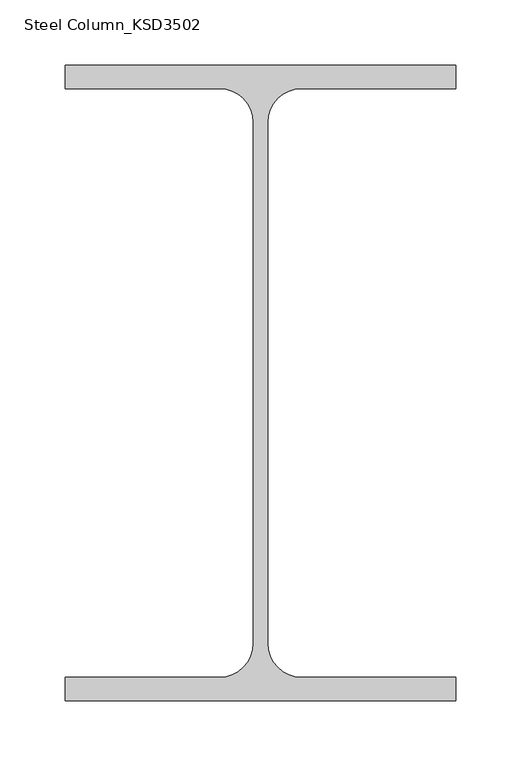
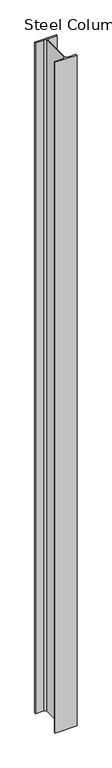
"""IFC4 building model written with IfcOpenShell, lengths in millimetres: column geometry, Steel Column_KSD3502 : H_SC_ASC_H-488×300x11x18."""

import ifcopenshell
import ifcopenshell.guid

model = None  # the IFC model being written
_history = None  # IfcOwnerHistory: only IFC2X3 demands one
_inside = {}  # id of a spatial element -> (the spatial element, [elements in it])
_under = {}  # id of a project, library or spatial element -> (it, [spatial elements below it])
_declared = {}  # id of a project -> (the project, [libraries it declares])
_typed = {}  # id of a type object -> (the type object, [elements of that type])
_made_of = {}  # id of a material, layer set ... -> (it, [elements and type objects made of it])


def new_model(schema):
    """Start an empty IFC model of exactly this schema.

    Asked for "IFC4X3", IfcOpenShell would pick the latest addendum, in which some entities
    have other attributes; the version numbers below select the first issue.
    IFC2X3 requires an IfcOwnerHistory on every rooted entity: one is made here for all.
    """
    global model, _history
    if schema == "IFC4X3":
        model = ifcopenshell.file(schema_version=(4, 3, 0, 0))
    else:
        model = ifcopenshell.file(schema=schema)
    _inside.clear()
    _under.clear()
    _declared.clear()
    _typed.clear()
    _made_of.clear()
    _history = None
    if model.schema == "IFC2X3":
        org = make("IfcOrganization", Name="unknown")
        user = make(
            "IfcPersonAndOrganization",
            ThePerson=make("IfcPerson", FamilyName="unknown"),
            TheOrganization=org,
        )
        app = make(
            "IfcApplication",
            ApplicationDeveloper=org,
            Version="unknown",
            ApplicationFullName="unknown",
            ApplicationIdentifier="unknown",
        )
        _history = make(
            "IfcOwnerHistory",
            OwningUser=user,
            OwningApplication=app,
            ChangeAction="ADDED",
            CreationDate=0,
        )
    return model


def make(cls, **values):
    """One entity of the class cls with the attributes given. An attribute that is None is left unset."""
    return model.create_entity(
        cls, **{name: value for name, value in values.items() if value is not None}
    )


def rooted(cls, **values):
    """An entity with a GlobalId (a new one), such as an element, a storey or a relation."""
    return make(cls, GlobalId=ifcopenshell.guid.new(), OwnerHistory=_history, **values)


def si_unit(unit_type, name, prefix=None):
    """IfcSIUnit, for example si_unit("LENGTHUNIT", "METRE", prefix="MILLI")."""
    return make("IfcSIUnit", UnitType=unit_type, Prefix=prefix, Name=name)


def assignment(units):
    """IfcUnitAssignment: the units of a project."""
    return None if units is None else make("IfcUnitAssignment", Units=units)


def point(xyz):
    """IfcCartesianPoint."""
    return None if xyz is None else make("IfcCartesianPoint", Coordinates=xyz)


def direction(xyz):
    """IfcDirection."""
    return None if xyz is None else make("IfcDirection", DirectionRatios=xyz)


def frame(location, z_axis=None, x_axis=None):
    """IfcAxis2Placement3D, a coordinate frame: its origin and axes. An axis left out is left unset."""
    return make(
        "IfcAxis2Placement3D",
        Location=point(location),
        Axis=direction(z_axis),
        RefDirection=direction(x_axis),
    )


def frame_2d(location, x_axis=None):
    """IfcAxis2Placement2D, a coordinate frame in the plane: its origin and x axis."""
    return make(
        "IfcAxis2Placement2D", Location=point(location), RefDirection=direction(x_axis)
    )


def origin():
    """The frame at (0, 0, 0) with its axes left unset."""
    return frame((0.0, 0.0, 0.0))


def place(relative_to, where):
    """IfcLocalPlacement: puts the frame where relative to a parent placement (None: the world)."""
    return make(
        "IfcLocalPlacement", PlacementRelTo=relative_to, RelativePlacement=where
    )


def context(
    kind, dimensions, precision=None, world=None, true_north=None, identifier=None
):
    """IfcGeometricRepresentationContext, for example the 3D "Model" context."""
    return make(
        "IfcGeometricRepresentationContext",
        ContextIdentifier=identifier,
        ContextType=kind,
        CoordinateSpaceDimension=dimensions,
        Precision=precision,
        WorldCoordinateSystem=world,
        TrueNorth=true_north,
    )


def project(units=None, contexts=None):
    """IfcProject with its units and contexts."""
    return rooted(
        "IfcProject",
        Name="project",
        RepresentationContexts=contexts,
        UnitsInContext=assignment(units),
    )


def spatial(cls, under=None, at=None, **own):
    """A site, building, storey or space (cls), placed at a placement, below another one or the project."""
    s = rooted(cls, ObjectPlacement=at, **own)
    if under is not None:
        _under.setdefault(under.id(), (under, []))[1].append(s)
    return s


def polyline(points):
    """IfcPolyline through the points."""
    return make("IfcPolyline", Points=[point(p) for p in points])


def circle_curve(where, radius):
    """IfcCircle in the frame where."""
    return make("IfcCircle", Position=where, Radius=radius)


def trimmed(basis, trim1, trim2, sense, master):
    """IfcTrimmedCurve: the piece of a basis curve between two trims."""
    return make(
        "IfcTrimmedCurve",
        BasisCurve=basis,
        Trim1=trim1,
        Trim2=trim2,
        SenseAgreement=sense,
        MasterRepresentation=master,
    )


def segment(curve, same_sense, transition):
    """IfcCompositeCurveSegment."""
    return make(
        "IfcCompositeCurveSegment",
        Transition=transition,
        SameSense=same_sense,
        ParentCurve=curve,
    )


def composite_curve(segments, self_intersect=None):
    """IfcCompositeCurve: segments joined end to end."""
    return make("IfcCompositeCurve", Segments=segments, SelfIntersect=self_intersect)


def outline(outer, holes=None, kind="AREA"):
    """IfcArbitraryClosedProfileDef: a profile drawn as a closed curve; with holes, ...WithVoids."""
    if holes is None:
        return make("IfcArbitraryClosedProfileDef", ProfileType=kind, OuterCurve=outer)
    return make(
        "IfcArbitraryProfileDefWithVoids",
        ProfileType=kind,
        OuterCurve=outer,
        InnerCurves=holes,
    )


def extrude(swept, where, along, depth):
    """IfcExtrudedAreaSolid: the profile swept, set in the frame where, extruded along a direction by depth."""
    return make(
        "IfcExtrudedAreaSolid",
        SweptArea=swept,
        Position=where,
        ExtrudedDirection=direction(along),
        Depth=depth,
    )


def shape(context_of_items, identifier, shape_type, items):
    """IfcShapeRepresentation: the items that make up one representation, for example the "Body"."""
    return make(
        "IfcShapeRepresentation",
        ContextOfItems=context_of_items,
        RepresentationIdentifier=identifier,
        RepresentationType=shape_type,
        Items=items,
    )


def source(mapping_origin, context_of_items, identifier, shape_type, items):
    """IfcRepresentationMap: a shape defined once, which mapped items show again and again."""
    return make(
        "IfcRepresentationMap",
        MappingOrigin=mapping_origin,
        MappedRepresentation=shape(context_of_items, identifier, shape_type, items),
    )


def transform(
    local_origin,
    x_axis=None,
    y_axis=None,
    z_axis=None,
    scale=None,
    scale2=None,
    scale3=None,
    uniform=True,
):
    """IfcCartesianTransformationOperator3D, or its non-uniform kind. x_axis, y_axis, z_axis: its Axis1, 2, 3."""
    if uniform:
        return make(
            "IfcCartesianTransformationOperator3D",
            Axis1=direction(x_axis),
            Axis2=direction(y_axis),
            LocalOrigin=point(local_origin),
            Scale=scale,
            Axis3=direction(z_axis),
        )
    return make(
        "IfcCartesianTransformationOperator3DnonUniform",
        Axis1=direction(x_axis),
        Axis2=direction(y_axis),
        LocalOrigin=point(local_origin),
        Scale=scale,
        Axis3=direction(z_axis),
        Scale2=scale2,
        Scale3=scale3,
    )


def mapped(mapping_source, mapping_target):
    """IfcMappedItem: shows the shape of a source again, moved by a transform."""
    return make(
        "IfcMappedItem", MappingSource=mapping_source, MappingTarget=mapping_target
    )


def made_of(thing, what):
    """Note that an element or type object is made of a material, layer set ...; save() writes the relation."""
    if what is not None:
        _made_of.setdefault(what.id(), (what, []))[1].append(thing)
    return thing


def element(
    cls,
    number,
    at=None,
    inside=None,
    cuts=None,
    type_object=None,
    material=None,
    context=None,
    identifier="Body",
    shape_type=None,
    held_by="IfcProductDefinitionShape",
    body=None,
    shapes=None,
    **own,
):
    """One element of the class cls, such as IfcWall. Its Tag is "e" and its number.

    at: its placement. inside: the storey or other place that contains it. cuts: it is an
    opening in that element (IfcRelVoidsElement). A single representation is given by context,
    identifier, shape_type and body (its items); several are given by shapes. held_by: the class
    of the entity that holds the representations. save() writes the other relations.
    """
    e = rooted(cls, Tag="e%d" % number, ObjectPlacement=at, **own)
    if body is not None:
        shapes = [shape(context, identifier, shape_type, body)]
    if shapes is not None:
        e.Representation = make(held_by, Representations=shapes)
    if inside is not None:
        _inside.setdefault(inside.id(), (inside, []))[1].append(e)
    if cuts is not None:
        rooted(
            "IfcRelVoidsElement", RelatingBuildingElement=cuts, RelatedOpeningElement=e
        )
    if type_object is not None:
        _typed.setdefault(type_object.id(), (type_object, []))[1].append(e)
    return made_of(e, material)


def aggregate(whole, parts):
    """IfcRelAggregates: a whole, such as a stair, and the parts it consists of."""
    return rooted("IfcRelAggregates", RelatingObject=whole, RelatedObjects=parts)


def save(model, path):
    """Write the relations noted so far, then the file.

    IfcRelAggregates (storeys below a building ...), IfcRelContainedInSpatialStructure (elements
    in a storey), IfcRelDefinesByType, IfcRelAssociatesMaterial and IfcRelDeclares: one each for
    every whole, place, type object, material and project.
    """
    for whole, parts in _under.values():
        aggregate(whole, parts)
    for where, things in _inside.values():
        rooted(
            "IfcRelContainedInSpatialStructure",
            RelatedElements=things,
            RelatingStructure=where,
        )
    for kind, things in _typed.values():
        rooted("IfcRelDefinesByType", RelatedObjects=things, RelatingType=kind)
    for what, things in _made_of.values():
        rooted("IfcRelAssociatesMaterial", RelatedObjects=things, RelatingMaterial=what)
    for by, libraries in _declared.values():
        rooted("IfcRelDeclares", RelatingContext=by, RelatedDefinitions=libraries)
    model.write(path)


def steel_column_ksd3502_bd22218f(model_context):
    return source(origin(), model_context, "Body", "SweptSolid", [
        extrude(outline(composite_curve([segment(polyline([(150.0, 244.0), (150.0, 226.0), (31.5, 226.0)]), True, "CONTINUOUS"), segment(trimmed(circle_curve(frame_2d((31.5, 200.0)), 26.0), [point((31.5, 226.0))], [point((5.5, 200.0))], True, "CARTESIAN"), True, "CONTINUOUS"), segment(polyline([(5.5, 200.0), (5.5, -200.0)]), True, "CONTINUOUS"), segment(trimmed(circle_curve(frame_2d((31.5, -200.0)), 26.0), [point((5.5, -200.0))], [point((31.5, -226.0))], True, "CARTESIAN"), True, "CONTINUOUS"), segment(polyline([(31.5, -226.0), (150.0, -226.0), (150.0, -244.0), (-150.0, -244.0), (-150.0, -226.0), (-31.5, -226.0)]), True, "CONTINUOUS"), segment(trimmed(circle_curve(frame_2d((-31.5, -200.0)), 26.0), [point((-31.5, -226.0))], [point((-5.5, -200.0))], True, "CARTESIAN"), True, "CONTINUOUS"), segment(polyline([(-5.5, -200.0), (-5.5, 200.0)]), True, "CONTINUOUS"), segment(trimmed(circle_curve(frame_2d((-31.5, 200.0)), 26.0), [point((-5.5, 200.0))], [point((-31.5, 226.0))], True, "CARTESIAN"), True, "CONTINUOUS"), segment(polyline([(-31.5, 226.0), (-150.0, 226.0), (-150.0, 244.0), (150.0, 244.0)]), True, "CONTINUOUS")], self_intersect=False)), frame((0.0, 0.0, 7538.9720055), z_axis=(0.0, 0.0, 1.0), x_axis=(1.0, 0.0, 0.0)), (0.0, 0.0, 1.0), 9761.0),
    ])


if __name__ == "__main__":
    model = new_model("IFC4")
    model_context = context("Model", 3, world=origin())
    ifc_project = project(units=[si_unit("LENGTHUNIT", "METRE", prefix="MILLI")], contexts=[model_context])
    site = spatial("IfcSite", under=ifc_project)
    building = spatial("IfcBuilding", under=site)
    placement = place(None, origin())
    steel_column_ksd3502_shape = steel_column_ksd3502_bd22218f(model_context)
    element("IfcColumn", 1, ObjectType="Steel Column_KSD3502 : H_SC_ASC_H-488×300x11x18", at=placement, inside=building, context=model_context, shape_type="MappedRepresentation", body=[
        mapped(steel_column_ksd3502_shape, transform((0.0, 0.0, 0.0), x_axis=(1.0, 0.0, 0.0), y_axis=(0.0, 1.0, 0.0), z_axis=(0.0, 0.0, 1.0))),
    ])
    save(model, "model.ifc")

# Revit data of these elements
# Type "Steel Column_KSD3502 : H_SC_ASC_H-488×300x11x18"
#   Width = 30.0 cm
#   Web Thickness = 1.1 cm
#   Web Fillet = 2.6 cm
#   Warping Constant = 4473230.0 cm⁶
#   Torsional Moment of Inertia = 137.492 cm⁴
#   Section Area = 163.5 cm²
#   Plastic Modulus weak axis = 830.0 cm³
#   Plastic Modulus strong axis = 3230.0 cm³
#   Perimeter = 1.27 m²/m
#   Nominal Weight = 128.00 kgf/m
#   Moment of Inertia weak axis = 8110.00 cm⁴
#   Moment of Inertia strong axis = 71000.00 cm⁴
#   Height = 48.8 cm
#   Flange Thickness = 1.8 cm
#   Elastic Modulus weak axis = 541.0 cm³
#   Elastic Modulus strong axis = 2910.0 cm³
#   Centroid Vertical = 24.4 cm
#   Centroid Horizontal = 15.0 cm
#   Bolt Spacing = 13.97 cm
#   Structural Material [instance default] = Steel, 45-345
#   Section Name Key = ""
#   Assembly Code = ""
# Element 1 (IfcColumn, "Steel Column_KSD3502 : H_SC_ASC_H-488×300x11x18")
#   Structural Material = none
# Materials
#   "Steel, 45-345": class "Metal", colour RGB 189 187 185, transparency 0, Description = "Steel 345 MPa", Cost = 0
